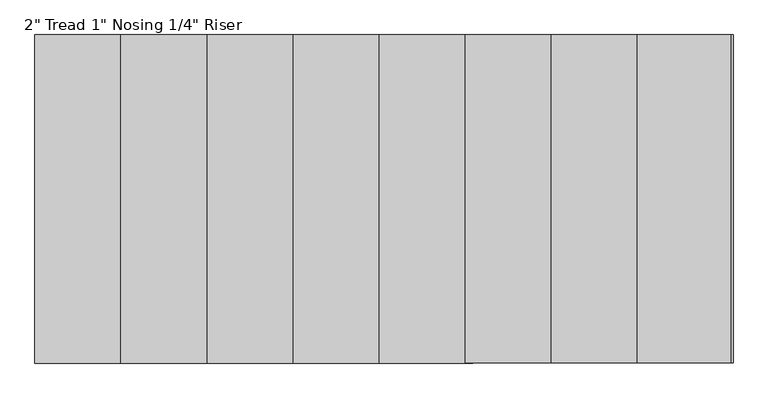
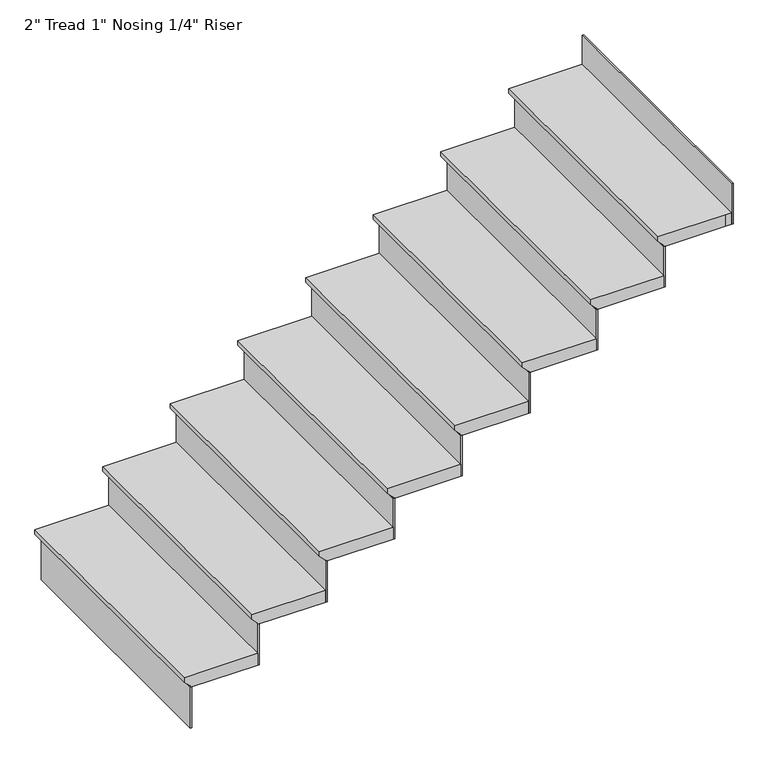
"""IFC4 building model written with IfcOpenShell, lengths in millimetres: stair flight geometry."""

import ifcopenshell
import ifcopenshell.guid

model = None  # the IFC model being written
_history = None  # IfcOwnerHistory: only IFC2X3 demands one
_inside = {}  # id of a spatial element -> (the spatial element, [elements in it])
_under = {}  # id of a project, library or spatial element -> (it, [spatial elements below it])
_declared = {}  # id of a project -> (the project, [libraries it declares])
_typed = {}  # id of a type object -> (the type object, [elements of that type])
_made_of = {}  # id of a material, layer set ... -> (it, [elements and type objects made of it])


def new_model(schema):
    """Start an empty IFC model of exactly this schema.

    Asked for "IFC4X3", IfcOpenShell would pick the latest addendum, in which some entities
    have other attributes; the version numbers below select the first issue.
    IFC2X3 requires an IfcOwnerHistory on every rooted entity: one is made here for all.
    """
    global model, _history
    if schema == "IFC4X3":
        model = ifcopenshell.file(schema_version=(4, 3, 0, 0))
    else:
        model = ifcopenshell.file(schema=schema)
    _inside.clear()
    _under.clear()
    _declared.clear()
    _typed.clear()
    _made_of.clear()
    _history = None
    if model.schema == "IFC2X3":
        org = make("IfcOrganization", Name="unknown")
        user = make(
            "IfcPersonAndOrganization",
            ThePerson=make("IfcPerson", FamilyName="unknown"),
            TheOrganization=org,
        )
        app = make(
            "IfcApplication",
            ApplicationDeveloper=org,
            Version="unknown",
            ApplicationFullName="unknown",
            ApplicationIdentifier="unknown",
        )
        _history = make(
            "IfcOwnerHistory",
            OwningUser=user,
            OwningApplication=app,
            ChangeAction="ADDED",
            CreationDate=0,
        )
    return model


def make(cls, **values):
    """One entity of the class cls with the attributes given. An attribute that is None is left unset."""
    return model.create_entity(
        cls, **{name: value for name, value in values.items() if value is not None}
    )


def rooted(cls, **values):
    """An entity with a GlobalId (a new one), such as an element, a storey or a relation."""
    return make(cls, GlobalId=ifcopenshell.guid.new(), OwnerHistory=_history, **values)


def si_unit(unit_type, name, prefix=None):
    """IfcSIUnit, for example si_unit("LENGTHUNIT", "METRE", prefix="MILLI")."""
    return make("IfcSIUnit", UnitType=unit_type, Prefix=prefix, Name=name)


def assignment(units):
    """IfcUnitAssignment: the units of a project."""
    return None if units is None else make("IfcUnitAssignment", Units=units)


def point(xyz):
    """IfcCartesianPoint."""
    return None if xyz is None else make("IfcCartesianPoint", Coordinates=xyz)


def direction(xyz):
    """IfcDirection."""
    return None if xyz is None else make("IfcDirection", DirectionRatios=xyz)


def frame(location, z_axis=None, x_axis=None):
    """IfcAxis2Placement3D, a coordinate frame: its origin and axes. An axis left out is left unset."""
    return make(
        "IfcAxis2Placement3D",
        Location=point(location),
        Axis=direction(z_axis),
        RefDirection=direction(x_axis),
    )


def origin():
    """The frame at (0, 0, 0) with its axes left unset."""
    return frame((0.0, 0.0, 0.0))


def place(relative_to, where):
    """IfcLocalPlacement: puts the frame where relative to a parent placement (None: the world)."""
    return make(
        "IfcLocalPlacement", PlacementRelTo=relative_to, RelativePlacement=where
    )


def context(
    kind, dimensions, precision=None, world=None, true_north=None, identifier=None
):
    """IfcGeometricRepresentationContext, for example the 3D "Model" context."""
    return make(
        "IfcGeometricRepresentationContext",
        ContextIdentifier=identifier,
        ContextType=kind,
        CoordinateSpaceDimension=dimensions,
        Precision=precision,
        WorldCoordinateSystem=world,
        TrueNorth=true_north,
    )


def project(units=None, contexts=None):
    """IfcProject with its units and contexts."""
    return rooted(
        "IfcProject",
        Name="project",
        RepresentationContexts=contexts,
        UnitsInContext=assignment(units),
    )


def spatial(cls, under=None, at=None, **own):
    """A site, building, storey or space (cls), placed at a placement, below another one or the project."""
    s = rooted(cls, ObjectPlacement=at, **own)
    if under is not None:
        _under.setdefault(under.id(), (under, []))[1].append(s)
    return s


def faces_of(points, faces, orient=None, outer=None):
    """IfcFace entities. A face is a list of loops; a loop is a list of indices into points, from 0.

    orient and outer hold one flag for each loop. By default every Orientation is true, the
    first loop of a face is its IfcFaceOuterBound and the others are IfcFaceBound.
    """
    made = []
    for i, loops in enumerate(faces):
        bounds = []
        for j, loop in enumerate(loops):
            is_outer = j == 0 if outer is None else outer[i][j]
            bounds.append(
                make(
                    "IfcFaceOuterBound" if is_outer else "IfcFaceBound",
                    Bound=make("IfcPolyLoop", Polygon=[points[k] for k in loop]),
                    Orientation=True if orient is None else orient[i][j],
                )
            )
        made.append(make("IfcFace", Bounds=bounds))
    return made


def faceted_brep(points, faces, orient=None, outer=None, voids=None):
    """IfcFacetedBrep: a solid bounded by flat faces; with voids (closed shells), ...WithVoids."""
    shared = [point(p) for p in points]
    hull = make("IfcClosedShell", CfsFaces=faces_of(shared, faces, orient, outer))
    if voids is None:
        return make("IfcFacetedBrep", Outer=hull)
    return make(
        "IfcFacetedBrepWithVoids",
        Outer=hull,
        Voids=[
            make(cls, CfsFaces=faces_of(shared, fs, o, b)) for cls, fs, o, b in voids
        ],
    )


def shape(context_of_items, identifier, shape_type, items):
    """IfcShapeRepresentation: the items that make up one representation, for example the "Body"."""
    return make(
        "IfcShapeRepresentation",
        ContextOfItems=context_of_items,
        RepresentationIdentifier=identifier,
        RepresentationType=shape_type,
        Items=items,
    )


def source(mapping_origin, context_of_items, identifier, shape_type, items):
    """IfcRepresentationMap: a shape defined once, which mapped items show again and again."""
    return make(
        "IfcRepresentationMap",
        MappingOrigin=mapping_origin,
        MappedRepresentation=shape(context_of_items, identifier, shape_type, items),
    )


def transform(
    local_origin,
    x_axis=None,
    y_axis=None,
    z_axis=None,
    scale=None,
    scale2=None,
    scale3=None,
    uniform=True,
):
    """IfcCartesianTransformationOperator3D, or its non-uniform kind. x_axis, y_axis, z_axis: its Axis1, 2, 3."""
    if uniform:
        return make(
            "IfcCartesianTransformationOperator3D",
            Axis1=direction(x_axis),
            Axis2=direction(y_axis),
            LocalOrigin=point(local_origin),
            Scale=scale,
            Axis3=direction(z_axis),
        )
    return make(
        "IfcCartesianTransformationOperator3DnonUniform",
        Axis1=direction(x_axis),
        Axis2=direction(y_axis),
        LocalOrigin=point(local_origin),
        Scale=scale,
        Axis3=direction(z_axis),
        Scale2=scale2,
        Scale3=scale3,
    )


def mapped(mapping_source, mapping_target):
    """IfcMappedItem: shows the shape of a source again, moved by a transform."""
    return make(
        "IfcMappedItem", MappingSource=mapping_source, MappingTarget=mapping_target
    )


def made_of(thing, what):
    """Note that an element or type object is made of a material, layer set ...; save() writes the relation."""
    if what is not None:
        _made_of.setdefault(what.id(), (what, []))[1].append(thing)
    return thing


def element(
    cls,
    number,
    at=None,
    inside=None,
    cuts=None,
    type_object=None,
    material=None,
    context=None,
    identifier="Body",
    shape_type=None,
    held_by="IfcProductDefinitionShape",
    body=None,
    shapes=None,
    **own,
):
    """One element of the class cls, such as IfcWall. Its Tag is "e" and its number.

    at: its placement. inside: the storey or other place that contains it. cuts: it is an
    opening in that element (IfcRelVoidsElement). A single representation is given by context,
    identifier, shape_type and body (its items); several are given by shapes. held_by: the class
    of the entity that holds the representations. save() writes the other relations.
    """
    e = rooted(cls, Tag="e%d" % number, ObjectPlacement=at, **own)
    if body is not None:
        shapes = [shape(context, identifier, shape_type, body)]
    if shapes is not None:
        e.Representation = make(held_by, Representations=shapes)
    if inside is not None:
        _inside.setdefault(inside.id(), (inside, []))[1].append(e)
    if cuts is not None:
        rooted(
            "IfcRelVoidsElement", RelatingBuildingElement=cuts, RelatedOpeningElement=e
        )
    if type_object is not None:
        _typed.setdefault(type_object.id(), (type_object, []))[1].append(e)
    return made_of(e, material)


def aggregate(whole, parts):
    """IfcRelAggregates: a whole, such as a stair, and the parts it consists of."""
    return rooted("IfcRelAggregates", RelatingObject=whole, RelatedObjects=parts)


def save(model, path):
    """Write the relations noted so far, then the file.

    IfcRelAggregates (storeys below a building ...), IfcRelContainedInSpatialStructure (elements
    in a storey), IfcRelDefinesByType, IfcRelAssociatesMaterial and IfcRelDeclares: one each for
    every whole, place, type object, material and project.
    """
    for whole, parts in _under.values():
        aggregate(whole, parts)
    for where, things in _inside.values():
        rooted(
            "IfcRelContainedInSpatialStructure",
            RelatedElements=things,
            RelatingStructure=where,
        )
    for kind, things in _typed.values():
        rooted("IfcRelDefinesByType", RelatedObjects=things, RelatingType=kind)
    for what, things in _made_of.values():
        rooted("IfcRelAssociatesMaterial", RelatedObjects=things, RelatingMaterial=what)
    for by, libraries in _declared.values():
        rooted("IfcRelDeclares", RelatingContext=by, RelatedDefinitions=libraries)
    model.write(path)


def stair_flight_9bc34bea(model_context):
    return source(origin(), model_context, "Body", "Brep", [
        faceted_brep([(663721.188677, -551651.2413841, 3346.1067568), (663721.188677, -551651.2413841, 3365.1567568), (663721.188677, -550584.4413841, 3365.1567568), (663721.188677, -550584.4413841, 3346.1067568), (663746.588677, -551651.2413841, 3320.7067568), (663746.588677, -550584.4413841, 3320.7067568), (664025.988677, -551651.2413841, 3365.1567568), (664025.988677, -550584.4413841, 3365.1567568), (663746.588677, -550584.4413841, 3314.3567568), (664025.988677, -550584.4413841, 3314.3567568), (664025.988677, -551651.2413841, 3314.3567568), (663746.588677, -551651.2413841, 3314.3567568)], [[[0, 1, 2, 3]], [[4, 0, 3, 5]], [[2, 1, 6, 7]], [[8, 9, 10, 11]], [[2, 7, 9, 8, 5, 3]], [[8, 11, 4, 5]], [[6, 1, 0, 4, 11, 10]], [[7, 6, 10, 9]]]),
        faceted_brep([(663746.588677, -551651.2413841, 3314.3567568), (663746.588677, -551651.2413841, 3137.2432432), (663752.938677, -551651.2413841, 3137.2432432), (663752.938677, -551651.2413841, 3314.3567568), (663746.588677, -550584.4413841, 3314.3567568), (663752.938677, -550584.4413841, 3314.3567568), (663752.938677, -550584.4413841, 3137.2432432), (663746.588677, -550584.4413841, 3137.2432432)], [[[0, 1, 2, 3]], [[4, 5, 6, 7]], [[1, 0, 4, 7]], [[2, 1, 7, 6]], [[3, 2, 6, 5]], [[0, 3, 5, 4]]]),
        faceted_brep([(664025.988677, -551651.2413841, 3491.4702703), (664025.988677, -551651.2413841, 3314.3567568), (664032.338677, -551651.2413841, 3314.3567568), (664032.338677, -551651.2413841, 3491.4702703), (664025.988677, -550584.4413841, 3491.4702703), (664032.338677, -550584.4413841, 3491.4702703), (664032.338677, -550584.4413841, 3314.3567568), (664025.988677, -550584.4413841, 3314.3567568)], [[[0, 1, 2, 3]], [[4, 5, 6, 7]], [[1, 0, 4, 7]], [[2, 1, 7, 6]], [[3, 2, 6, 5]], [[0, 3, 5, 4]]]),
        faceted_brep([(664000.588677, -550584.4413841, 3542.2702703), (664000.588677, -551651.2413841, 3542.2702703), (664305.388677, -551651.2413841, 3542.2702703), (664305.388677, -550584.4413841, 3542.2702703), (664025.988677, -550584.4413841, 3491.4702703), (664305.388677, -550584.4413841, 3491.4702703), (664305.388677, -551651.2413841, 3491.4702703), (664025.988677, -551651.2413841, 3491.4702703), (664025.988677, -550584.4413841, 3497.8202703), (664000.588677, -550584.4413841, 3523.2202703), (664025.988677, -551651.2413841, 3497.8202703), (664000.588677, -551651.2413841, 3523.2202703)], [[[0, 1, 2, 3]], [[4, 5, 6, 7]], [[0, 3, 5, 4, 8, 9]], [[4, 7, 10, 8]], [[2, 1, 11, 10, 7, 6]], [[3, 2, 6, 5]], [[11, 1, 0, 9]], [[10, 11, 9, 8]]]),
        faceted_brep([(664305.388677, -551651.2413841, 3668.5837838), (664305.388677, -551651.2413841, 3491.4702703), (664311.738677, -551651.2413841, 3491.4702703), (664311.738677, -551651.2413841, 3668.5837838), (664305.388677, -550584.4413841, 3668.5837838), (664311.738677, -550584.4413841, 3668.5837838), (664311.738677, -550584.4413841, 3491.4702703), (664305.388677, -550584.4413841, 3491.4702703)], [[[0, 1, 2, 3]], [[4, 5, 6, 7]], [[1, 0, 4, 7]], [[2, 1, 7, 6]], [[3, 2, 6, 5]], [[0, 3, 5, 4]]]),
        faceted_brep([(664279.988677, -550584.4413841, 3719.3837838), (664279.988677, -551651.2413841, 3719.3837838), (664584.788677, -551651.2413841, 3719.3837838), (664584.788677, -550584.4413841, 3719.3837838), (664305.388677, -550584.4413841, 3668.5837838), (664584.788677, -550584.4413841, 3668.5837838), (664584.788677, -551651.2413841, 3668.5837838), (664305.388677, -551651.2413841, 3668.5837838), (664305.388677, -550584.4413841, 3674.9337838), (664279.988677, -550584.4413841, 3700.3337838), (664305.388677, -551651.2413841, 3674.9337838), (664279.988677, -551651.2413841, 3700.3337838)], [[[0, 1, 2, 3]], [[4, 5, 6, 7]], [[0, 3, 5, 4, 8, 9]], [[4, 7, 10, 8]], [[2, 1, 11, 10, 7, 6]], [[3, 2, 6, 5]], [[11, 1, 0, 9]], [[10, 11, 9, 8]]]),
        faceted_brep([(664584.788677, -551651.2413841, 3845.6972973), (664584.788677, -551651.2413841, 3668.5837838), (664591.138677, -551651.2413841, 3668.5837838), (664591.138677, -551651.2413841, 3845.6972973), (664584.788677, -550584.4413841, 3845.6972973), (664591.138677, -550584.4413841, 3845.6972973), (664591.138677, -550584.4413841, 3668.5837838), (664584.788677, -550584.4413841, 3668.5837838)], [[[0, 1, 2, 3]], [[4, 5, 6, 7]], [[1, 0, 4, 7]], [[2, 1, 7, 6]], [[3, 2, 6, 5]], [[0, 3, 5, 4]]]),
        faceted_brep([(664559.388677, -550584.4413841, 3896.4972973), (664559.388677, -551651.2413841, 3896.4972973), (664864.188677, -551651.2413841, 3896.4972973), (664864.188677, -550584.4413841, 3896.4972973), (664584.788677, -550584.4413841, 3845.6972973), (664864.188677, -550584.4413841, 3845.6972973), (664864.188677, -551651.2413841, 3845.6972973), (664584.788677, -551651.2413841, 3845.6972973), (664584.788677, -550584.4413841, 3852.0472973), (664559.388677, -550584.4413841, 3877.4472973), (664584.788677, -551651.2413841, 3852.0472973), (664559.388677, -551651.2413841, 3877.4472973)], [[[0, 1, 2, 3]], [[4, 5, 6, 7]], [[0, 3, 5, 4, 8, 9]], [[4, 7, 10, 8]], [[2, 1, 11, 10, 7, 6]], [[3, 2, 6, 5]], [[11, 1, 0, 9]], [[10, 11, 9, 8]]]),
        faceted_brep([(664864.188677, -551651.2413841, 4022.8108108), (664864.188677, -551651.2413841, 3845.6972973), (664870.538677, -551651.2413841, 3845.6972973), (664870.538677, -551651.2413841, 4022.8108108), (664864.188677, -550584.4413841, 4022.8108108), (664870.538677, -550584.4413841, 4022.8108108), (664870.538677, -550584.4413841, 3845.6972973), (664864.188677, -550584.4413841, 3845.6972973)], [[[0, 1, 2, 3]], [[4, 5, 6, 7]], [[1, 0, 4, 7]], [[2, 1, 7, 6]], [[3, 2, 6, 5]], [[0, 3, 5, 4]]]),
        faceted_brep([(664838.788677, -550584.4413841, 4073.6108108), (664838.788677, -551651.2413841, 4073.6108108), (665143.588677, -551651.2413841, 4073.6108108), (665143.588677, -550584.4413841, 4073.6108108), (664864.188677, -550584.4413841, 4022.8108108), (665143.588677, -550584.4413841, 4022.8108108), (665143.588677, -551651.2413841, 4022.8108108), (664864.188677, -551651.2413841, 4022.8108108), (664864.188677, -550584.4413841, 4029.1608108), (664838.788677, -550584.4413841, 4054.5608108), (664864.188677, -551651.2413841, 4029.1608108), (664838.788677, -551651.2413841, 4054.5608108)], [[[0, 1, 2, 3]], [[4, 5, 6, 7]], [[0, 3, 5, 4, 8, 9]], [[4, 7, 10, 8]], [[2, 1, 11, 10, 7, 6]], [[3, 2, 6, 5]], [[11, 1, 0, 9]], [[10, 11, 9, 8]]]),
        faceted_brep([(665143.588677, -551651.2413841, 4199.9243243), (665143.588677, -551651.2413841, 4022.8108108), (665149.938677, -551651.2413841, 4022.8108108), (665149.938677, -551651.2413841, 4199.9243243), (665143.588677, -550584.4413841, 4199.9243243), (665149.938677, -550584.4413841, 4199.9243243), (665149.938677, -550584.4413841, 4022.8108108), (665143.588677, -550584.4413841, 4022.8108108)], [[[0, 1, 2, 3]], [[4, 5, 6, 7]], [[1, 0, 4, 7]], [[2, 1, 7, 6]], [[3, 2, 6, 5]], [[0, 3, 5, 4]]]),
        faceted_brep([(665118.188677, -550584.4413841, 4250.7243243), (665118.188677, -551651.2413841, 4250.7243243), (665422.988677, -551651.2413841, 4250.7243243), (665422.988677, -550584.4413841, 4250.7243243), (665143.588677, -550584.4413841, 4199.9243243), (665422.988677, -550584.4413841, 4199.9243243), (665422.988677, -551651.2413841, 4199.9243243), (665143.588677, -551651.2413841, 4199.9243243), (665143.588677, -550584.4413841, 4206.2743243), (665118.188677, -550584.4413841, 4231.6743243), (665143.588677, -551651.2413841, 4206.2743243), (665118.188677, -551651.2413841, 4231.6743243)], [[[0, 1, 2, 3]], [[4, 5, 6, 7]], [[0, 3, 5, 4, 8, 9]], [[4, 7, 10, 8]], [[2, 1, 11, 10, 7, 6]], [[3, 2, 6, 5]], [[11, 1, 0, 9]], [[10, 11, 9, 8]]]),
        faceted_brep([(665422.988677, -551651.2413841, 4377.0378378), (665422.988677, -551651.2413841, 4199.9243243), (665429.338677, -551651.2413841, 4199.9243243), (665429.338677, -551651.2413841, 4377.0378378), (665422.988677, -550584.4413841, 4377.0378378), (665429.338677, -550584.4413841, 4377.0378378), (665429.338677, -550584.4413841, 4199.9243243), (665422.988677, -550584.4413841, 4199.9243243)], [[[0, 1, 2, 3]], [[4, 5, 6, 7]], [[1, 0, 4, 7]], [[2, 1, 7, 6]], [[3, 2, 6, 5]], [[0, 3, 5, 4]]]),
        faceted_brep([(665397.588677, -550584.4413841, 4427.8378378), (665397.588677, -551651.2413841, 4427.8378378), (665702.388677, -551651.2413841, 4427.8378378), (665702.388677, -550584.4413841, 4427.8378378), (665422.988677, -550584.4413841, 4377.0378378), (665702.388677, -550584.4413841, 4377.0378378), (665702.388677, -551651.2413841, 4377.0378378), (665422.988677, -551651.2413841, 4377.0378378), (665422.988677, -550584.4413841, 4383.3878378), (665397.588677, -550584.4413841, 4408.7878378), (665422.988677, -551651.2413841, 4383.3878378), (665397.588677, -551651.2413841, 4408.7878378)], [[[0, 1, 2, 3]], [[4, 5, 6, 7]], [[0, 3, 5, 4, 8, 9]], [[4, 7, 10, 8]], [[2, 1, 11, 10, 7, 6]], [[3, 2, 6, 5]], [[11, 1, 0, 9]], [[10, 11, 9, 8]]]),
        faceted_brep([(665981.788677, -551651.2413841, 4731.2648649), (665981.788677, -551651.2413841, 4554.1513514), (665988.138677, -551651.2413841, 4554.1513514), (665988.138677, -551651.2413841, 4731.2648649), (665981.788677, -550584.4413841, 4731.2648649), (665988.138677, -550584.4413841, 4731.2648649), (665988.138677, -550584.4413841, 4554.1513514), (665981.788677, -550584.4413841, 4554.1513514)], [[[0, 1, 2, 3]], [[4, 5, 6, 7]], [[1, 0, 4, 7]], [[2, 1, 7, 6]], [[3, 2, 6, 5]], [[0, 3, 5, 4]]]),
        faceted_brep([(665702.388677, -551651.2413841, 4554.1513514), (665702.388677, -551651.2413841, 4377.0378378), (665708.738677, -551651.2413841, 4377.0378378), (665708.738677, -551651.2413841, 4554.1513514), (665702.388677, -550584.4413841, 4554.1513514), (665708.738677, -550584.4413841, 4554.1513514), (665708.738677, -550584.4413841, 4377.0378378), (665702.388677, -550584.4413841, 4377.0378378)], [[[0, 1, 2, 3]], [[4, 5, 6, 7]], [[1, 0, 4, 7]], [[2, 1, 7, 6]], [[3, 2, 6, 5]], [[0, 3, 5, 4]]]),
        faceted_brep([(665676.988677, -550584.4413841, 4604.9513514), (665676.988677, -551651.2413841, 4604.9513514), (665956.388677, -551651.2413841, 4604.9513514), (665981.788677, -551651.2413841, 4604.9513514), (665981.788677, -550584.4413841, 4604.9513514), (665702.388677, -550584.4413841, 4554.1513514), (665981.788677, -550584.4413841, 4554.1513514), (665981.788677, -551651.2413841, 4554.1513514), (665956.388677, -551651.2413841, 4554.1513514), (665702.388677, -551651.2413841, 4554.1513514), (665702.388677, -550584.4413841, 4560.5013514), (665676.988677, -550584.4413841, 4585.9013514), (665702.388677, -551651.2413841, 4560.5013514), (665676.988677, -551651.2413841, 4585.9013514)], [[[0, 1, 2, 3, 4]], [[5, 6, 7, 8, 9]], [[0, 4, 6, 5, 10, 11]], [[5, 9, 12, 10]], [[2, 1, 13, 12, 9, 8]], [[3, 2, 8, 7]], [[4, 3, 7, 6]], [[13, 1, 0, 11]], [[12, 13, 11, 10]]]),
    ])


if __name__ == "__main__":
    model = new_model("IFC4")
    model_context = context("Model", 3, world=origin())
    ifc_project = project(units=[si_unit("LENGTHUNIT", "METRE", prefix="MILLI")], contexts=[model_context])
    site = spatial("IfcSite", under=ifc_project)
    building = spatial("IfcBuilding", under=site)
    placement = place(None, origin())
    stair_flight_shape = stair_flight_9bc34bea(model_context)
    element("IfcStairFlight", 1, ObjectType="2\" Tread 1\" Nosing 1/4\" Riser", at=placement, inside=building, context=model_context, shape_type="MappedRepresentation", body=[
        mapped(stair_flight_shape, transform((0.0, 0.0, 0.0), x_axis=(1.0, 0.0, 0.0), y_axis=(0.0, 1.0, 0.0), z_axis=(0.0, 0.0, 1.0))),
    ])
    save(model, "model.ifc")
